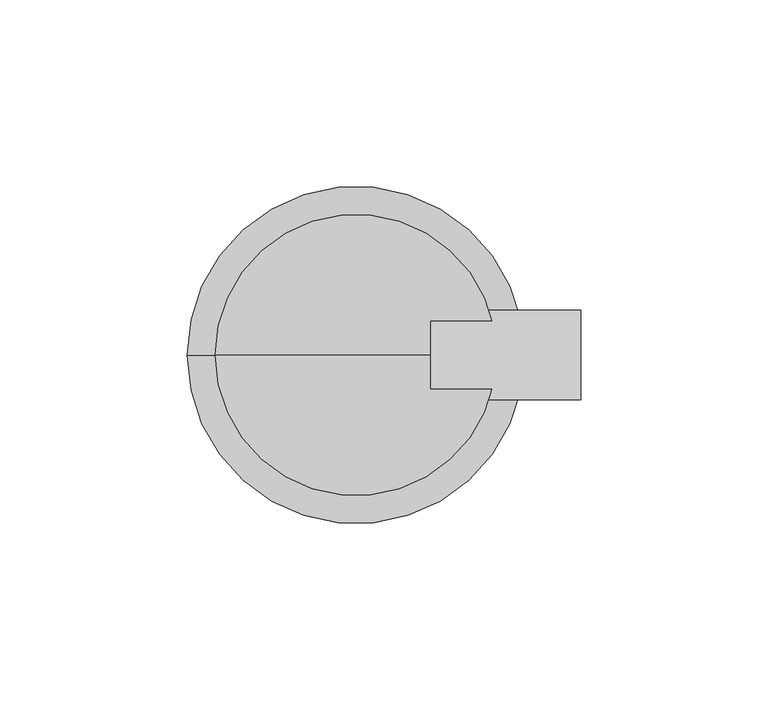
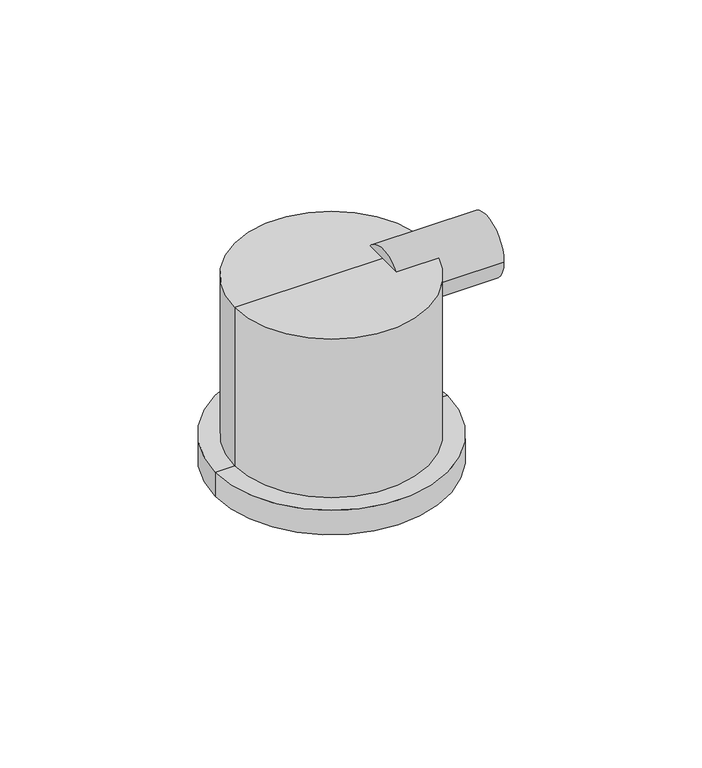
"""IFC4 building model written with IfcOpenShell, lengths in millimetres: proxy geometry, SE_SPP_Pressure relay : SPP930-2200."""

from ifc_helpers import new_model, si_unit, point, frame, frame_2d, origin, place, context, project, spatial, circle_curve, trimmed, segment, composite_curve, outline, extrude, source, transform, mapped, element, save
from ifc_brep_helpers import plane_surface, cylinder_surface, advanced_brep


def generic_models_16f3a452(model_context):
    return source(origin(), model_context, "Body", "SolidModel", [
        extrude(outline(composite_curve([segment(trimmed(circle_curve(frame_2d((0.0, 76.6713082)), 12.0), [point((-12.0, 76.6713082))], [point((12.0, 76.6713082))], False, "CARTESIAN"), True, "CONTINUOUS"), segment(trimmed(circle_curve(frame_2d((0.0, 76.6713082)), 12.0), [point((12.0, 76.6713082))], [point((-12.0, 76.6713082))], False, "CARTESIAN"), True, "CONTINUOUS")], self_intersect=False)), frame((20.0, 0.0, 0.0), z_axis=(1.0, 0.0, 0.0), x_axis=(0.0, 1.0, 0.0)), (0.0, 0.0, 1.0), 40.0),
        advanced_brep(
        [(0.0, 0.0, -13.0430706), (-10.0, 0.0, -13.0430706), (10.0, 0.0, -13.0430706), (37.5, 0.0, 84.9569294), (-37.5, 0.0, 84.9569294), (0.0, 0.0, 84.9569294), (37.5, 0.0, 20.0), (-37.5, 0.0, 20.0), (45.0, 0.0, 20.0), (-45.0, 0.0, 20.0), (45.0, 0.0, 10.0), (-45.0, 0.0, 10.0), (10.0, 0.0, 10.0), (-10.0, 0.0, 10.0), (10.0, 0.0, 0.0), (-10.0, 0.0, 0.0)],
        [
            (0, 1),
            (1, 2, circle_curve(frame((0.0, 0.0, -13.0430706), z_axis=(0.0, 0.0, -1.0), x_axis=(-1.0, 0.0, 0.0)), 10.0)),
            (2, 0),
            (2, 1, circle_curve(frame((0.0, 0.0, -13.0430706), z_axis=(0.0, 0.0, -1.0), x_axis=(-1.0, 0.0, 0.0)), 10.0)),
            (3, 4, circle_curve(frame((0.0, 0.0, 84.9569294), z_axis=(0.0, 0.0, 1.0), x_axis=(-1.0, 0.0, 0.0)), 37.5)),
            (4, 5),
            (5, 3),
            (4, 3, circle_curve(frame((0.0, 0.0, 84.9569294), z_axis=(0.0, 0.0, 1.0), x_axis=(-1.0, 0.0, 0.0)), 37.5)),
            (6, 7, circle_curve(frame((0.0, 0.0, 20.0), z_axis=(0.0, 0.0, 1.0), x_axis=(-1.0, 0.0, 0.0)), 37.5)),
            (7, 4),
            (3, 6),
            (7, 6, circle_curve(frame((0.0, 0.0, 20.0), z_axis=(0.0, 0.0, 1.0), x_axis=(-1.0, 0.0, 0.0)), 37.5)),
            (8, 9, circle_curve(frame((0.0, 0.0, 20.0), z_axis=(0.0, 0.0, 1.0), x_axis=(-1.0, 0.0, 0.0)), 45.0)),
            (9, 7),
            (6, 8),
            (9, 8, circle_curve(frame((0.0, 0.0, 20.0), z_axis=(0.0, 0.0, 1.0), x_axis=(-1.0, 0.0, 0.0)), 45.0)),
            (10, 11, circle_curve(frame((0.0, 0.0, 10.0), z_axis=(0.0, 0.0, 1.0), x_axis=(-1.0, 0.0, 0.0)), 45.0)),
            (11, 9),
            (8, 10),
            (11, 10, circle_curve(frame((0.0, 0.0, 10.0), z_axis=(0.0, 0.0, 1.0), x_axis=(-1.0, 0.0, 0.0)), 45.0)),
            (12, 13, circle_curve(frame((0.0, 0.0, 10.0), z_axis=(0.0, 0.0, 1.0), x_axis=(-1.0, 0.0, 0.0)), 10.0)),
            (13, 11),
            (10, 12),
            (13, 12, circle_curve(frame((0.0, 0.0, 10.0), z_axis=(0.0, 0.0, 1.0), x_axis=(-1.0, 0.0, 0.0)), 10.0)),
            (14, 15, circle_curve(frame((0.0, 0.0, 0.0), z_axis=(0.0, 0.0, 1.0), x_axis=(-1.0, 0.0, 0.0)), 10.0)),
            (15, 13),
            (12, 14),
            (15, 14, circle_curve(frame((0.0, 0.0, 0.0), z_axis=(0.0, 0.0, 1.0), x_axis=(-1.0, 0.0, 0.0)), 10.0)),
            (1, 15),
            (14, 2),
        ],
        [
            plane_surface(frame((0.0, 0.0, -13.0430706), z_axis=(0.0, 0.0, -1.0), x_axis=(-1.0, 0.0, 0.0))),
            plane_surface(frame((0.0, 0.0, 84.9569294), z_axis=(0.0, 0.0, 1.0), x_axis=(-1.0, 0.0, 0.0))),
            cylinder_surface(frame((0.0, 0.0, 470.2928861), z_axis=(0.0, 0.0, -1.0), x_axis=(-1.0, 0.0, 0.0)), 37.5),
            plane_surface(frame((0.0, 0.0, 20.0), z_axis=(0.0, 0.0, 1.0), x_axis=(-1.0, 0.0, 0.0))),
            cylinder_surface(frame((0.0, 0.0, 470.2928861), z_axis=(0.0, 0.0, -1.0), x_axis=(-1.0, 0.0, 0.0)), 45.0),
            plane_surface(frame((0.0, 0.0, 10.0), z_axis=(0.0, 0.0, -1.0), x_axis=(-1.0, 0.0, 0.0))),
            cylinder_surface(frame((0.0, 0.0, 470.2928861), z_axis=(0.0, 0.0, -1.0), x_axis=(-1.0, 0.0, 0.0)), 10.0),
        ],
        [
            (0, [[1, 2, 3]]),
            (0, [[-3, 4, -1]]),
            (1, [[5, 6, 7]]),
            (1, [[8, -7, -6]]),
            (2, [[9, 10, -5, 11]]),
            (2, [[12, -11, -8, -10]]),
            (3, [[13, 14, -9, 15]]),
            (3, [[16, -15, -12, -14]]),
            (4, [[17, 18, -13, 19]]),
            (4, [[20, -19, -16, -18]]),
            (5, [[21, 22, -17, 23]]),
            (5, [[24, -23, -20, -22]]),
            (6, [[25, 26, -21, 27]]),
            (6, [[28, -27, -24, -26]]),
            (6, [[-2, 29, -25, 30]]),
            (6, [[-4, -30, -28, -29]]),
        ],
    ),
    ])


if __name__ == "__main__":
    model = new_model("IFC4")
    model_context = context("Model", 3, world=origin())
    ifc_project = project(units=[si_unit("LENGTHUNIT", "METRE", prefix="MILLI")], contexts=[model_context])
    site = spatial("IfcSite", under=ifc_project)
    building = spatial("IfcBuilding", under=site)
    placement = place(None, origin())
    generic_models_shape = generic_models_16f3a452(model_context)
    element("IfcBuildingElementProxy", 1, Name="SE_SPP_Pressure relay : SPP930-2200", ObjectType="SE_SPP_Pressure relay : SPP930-2200", at=placement, inside=building, context=model_context, shape_type="MappedRepresentation", body=[
        mapped(generic_models_shape, transform((0.0, 0.0, 0.0), x_axis=(1.0, 0.0, 0.0), y_axis=(0.0, 1.0, 0.0), z_axis=(0.0, 0.0, 1.0))),
    ])
    save(model, "model.ifc")

# Revit data of these elements
# Project information
#   Наименование здания = "Наименование здания"
#   Дата утверждения проекта = "Дата"
#   Статус проекта = "П"
#   Заказчик = "Заказчик"
#   Адрес проекта = "Адрес проекта"
#   Наименование проекта = "Наименование проекта"
#   Номер проекта = "Номер проекта"
# Type "SE_SPP_Pressure relay : SPP930-2200"
#   ADSK_Предел огнестойкости = ""
#   ADSK_Обозначение [instance default] = ""
#   ADSK_Наименование краткое = ""
#   ADSK_Наименование = "Реле давления жидкости/воздуха SPP930-2200, IP54, 0,12-2,2бар"
#   ADSK_Марка = "SPP930-2200"
#   ADSK_Код изделия = "004701160"
#   ADSK_Завод-изготовитель = "Schneider Electric"
#   ADSK_Единица измерения = "шт."
#   КЛ_Ширина [instance default] = 0 mm
#   КЛ_Высота [instance default] = 0 mm
#   К_Диаметр [instance default] = 0 mm
#   SE_Минимальная температура работы = -10 °C
#   SE_Максимальная температура работы = 80 °C
#   ADSK_Ток = 0 A
#   ADSK_Размер_Ширина = 58.5 mm
#   ADSK_Размер_Смещение от уровня [instance default] = 0 mm
#   ADSK_Размер_Глубина = 58.5 mm
#   ADSK_Размер_Высота = 98 mm
#   ADSK_Полная мощность = 0 VA
#   ADSK_Номинальная мощность = 0 W
#   ADSK_Напряжение = 24 V
#   ADSK_Масса = 0
#   ADSK_Коэффициент мощности = 1
#   ADSK_Количество [instance default] = 1
#   ADSK_Количество фаз = 3
#   ADSK_Классификация нагрузок [instance default] = Датчик давления
#   Default Elevation = 0
